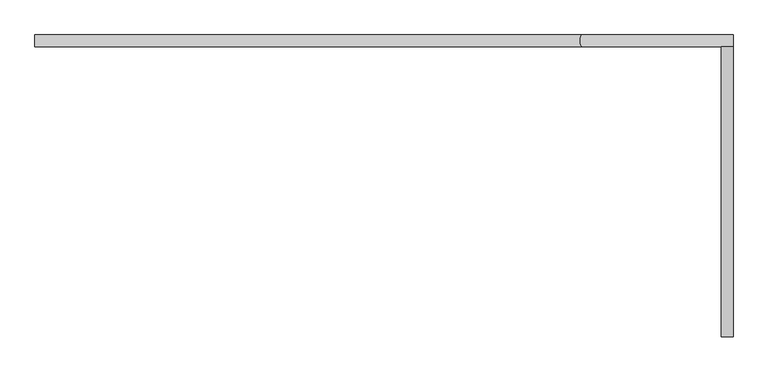
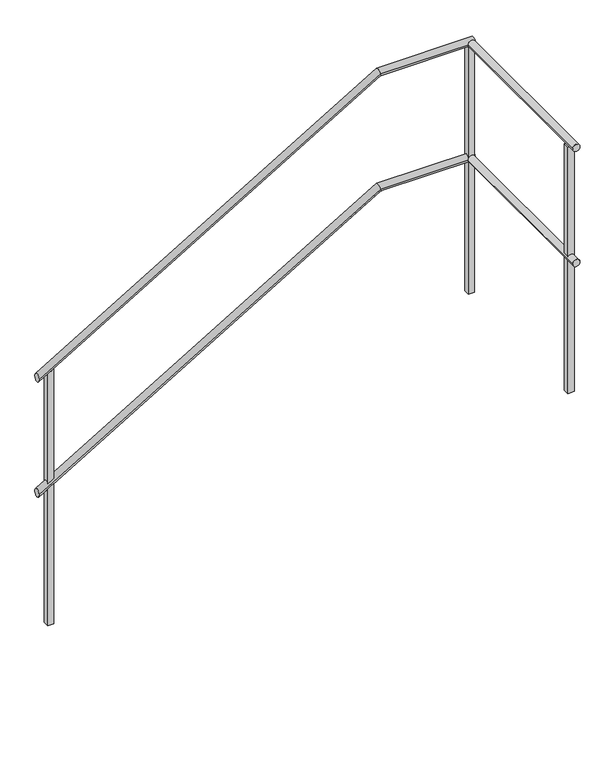
"""IFC4 building model written with IfcOpenShell, lengths in millimetres: railing geometry."""

from ifc_helpers import new_model, si_unit, frame, origin, place, context, project, spatial, polyline, circle_curve, ellipse_curve, outline, extrude, source, transform, mapped, element, save
from ifc_brep_helpers import plane_surface, cylinder_surface, advanced_brep


def railing_ac14cb65(model_context):
    return source(origin(), model_context, "Body", "SolidModel", [
        advanced_brep(
        [(43964.6, 23749.5208589, 1734.9618634), (43994.6, 23749.5208589, 1734.9618634), (43964.6, 24494.1208589, 1734.9618634), (43994.6, 24494.1208589, 1734.9618634)],
        [
            (0, 1, circle_curve(frame((43979.6, 23749.5208589, 1734.9618634), z_axis=(0.0, -1.0, 0.0), x_axis=(1.0, 0.0, 0.0)), 15.0)),
            (1, 0, circle_curve(frame((43979.6, 23749.5208589, 1734.9618634), z_axis=(0.0, -1.0, 0.0), x_axis=(1.0, 0.0, 0.0)), 15.0)),
            (2, 3, circle_curve(frame((43979.6, 24494.1208589, 1734.9618634), z_axis=(0.0, 1.0, 0.0), x_axis=(1.0, 0.0, 0.0)), 15.0)),
            (3, 2, circle_curve(frame((43979.6, 24494.1208589, 1734.9618634), z_axis=(0.0, 1.0, 0.0), x_axis=(1.0, 0.0, 0.0)), 15.0)),
            (0, 2),
            (3, 1),
        ],
        [
            plane_surface(frame((43979.6, 23749.5208589, 1749.9618634), z_axis=(0.0, -1.0, 0.0), x_axis=(0.0, 0.0, 1.0))),
            plane_surface(frame((43979.6, 24494.1208589, 1749.9618634), z_axis=(0.0, 1.0, 0.0), x_axis=(0.0, 0.0, 1.0))),
            cylinder_surface(frame((43979.6, 23749.5208589, 1734.9618634), z_axis=(0.0, -1.0, 0.0), x_axis=(1.0, 0.0, 0.0)), 15.0),
        ],
        [
            (0, [[1, 2]]),
            (1, [[3, 4]]),
            (2, [[-1, 5, -4, 6]]),
            (2, [[-2, -6, -3, -5]]),
        ],
    ),
        advanced_brep(
        [(43994.6, 24494.1208589, 1734.9618634), (43994.6, 24524.1208589, 1734.9618634), (43606.242552, 24494.1208589, 1734.9618634), (43606.242552, 24524.1208589, 1734.9618634), (42202.1161135, 24494.1208589, 899.1723166), (42202.1161135, 24524.1208589, 899.1723166)],
        [
            (0, 1, circle_curve(frame((43994.6, 24509.1208589, 1734.9618634), z_axis=(1.0, 0.0, 0.0), x_axis=(0.0, 1.0, 0.0)), 15.0)),
            (1, 0, circle_curve(frame((43994.6, 24509.1208589, 1734.9618634), z_axis=(1.0, 0.0, 0.0), x_axis=(0.0, 1.0, 0.0)), 15.0)),
            (0, 2),
            (2, 3, ellipse_curve(frame((43606.242552, 24509.1208589, 1734.9618634), z_axis=(0.9641817474962143, 0.0, 0.26524245096731114), x_axis=(0.265242450967311, 0.0, -0.9641817474962145)), 15.5572329, 15.0)),
            (3, 1),
            (3, 2, ellipse_curve(frame((43606.242552, 24509.1208589, 1734.9618634), z_axis=(0.9641817474962143, 0.0, 0.26524245096731114), x_axis=(0.265242450967311, 0.0, -0.9641817474962145)), 15.5572329, 15.0)),
            (4, 5, ellipse_curve(frame((42202.1161135, 24509.1208589, 899.1723166), z_axis=(-1.0, 0.0, 0.0), x_axis=(0.0, 0.0, 1.0)), 17.4562134, 15.0)),
            (5, 4, ellipse_curve(frame((42202.1161135, 24509.1208589, 899.1723166), z_axis=(-1.0, 0.0, 0.0), x_axis=(0.0, 0.0, 1.0)), 17.4562134, 15.0)),
            (2, 4),
            (5, 3),
        ],
        [
            plane_surface(frame((43994.6, 24509.1208589, 1749.9618634), z_axis=(1.0, 0.0, 0.0), x_axis=(0.0, -1.0, 0.0))),
            cylinder_surface(frame((43994.6, 24509.1208589, 1734.9618634), z_axis=(1.0, 0.0, 0.0), x_axis=(0.0, 1.0, 0.0)), 15.0),
            plane_surface(frame((42202.1161135, 24509.1208589, 916.62853), z_axis=(-1.0, 0.0, 0.0), x_axis=(0.0, -1.0, 0.0))),
            cylinder_surface(frame((43609.7883714, 24509.1208589, 1737.0724701), z_axis=(0.8592928844097072, 0.0, 0.511483859767682), x_axis=(0.0, 1.0, 0.0)), 15.0),
        ],
        [
            (0, [[1, 2]]),
            (1, [[-1, 3, 4, 5]]),
            (1, [[-2, -5, 6, -3]]),
            (2, [[7, 8]]),
            (3, [[-4, 9, -8, 10]]),
            (3, [[-6, -10, -7, -9]]),
        ],
    ),
        advanced_brep(
        [(43964.6, 23749.5208589, 2234.9618634), (43994.6, 23749.5208589, 2234.9618634), (43964.6, 24494.1208589, 2234.9618634), (43994.6, 24494.1208589, 2234.9618634)],
        [
            (0, 1, circle_curve(frame((43979.6, 23749.5208589, 2234.9618634), z_axis=(0.0, -1.0, 0.0), x_axis=(1.0, 0.0, 0.0)), 15.0)),
            (1, 0, circle_curve(frame((43979.6, 23749.5208589, 2234.9618634), z_axis=(0.0, -1.0, 0.0), x_axis=(1.0, 0.0, 0.0)), 15.0)),
            (2, 3, circle_curve(frame((43979.6, 24494.1208589, 2234.9618634), z_axis=(0.0, 1.0, 0.0), x_axis=(1.0, 0.0, 0.0)), 15.0)),
            (3, 2, circle_curve(frame((43979.6, 24494.1208589, 2234.9618634), z_axis=(0.0, 1.0, 0.0), x_axis=(1.0, 0.0, 0.0)), 15.0)),
            (0, 2),
            (3, 1),
        ],
        [
            plane_surface(frame((43979.6, 23749.5208589, 2249.9618634), z_axis=(0.0, -1.0, 0.0), x_axis=(0.0, 0.0, 1.0))),
            plane_surface(frame((43979.6, 24494.1208589, 2249.9618634), z_axis=(0.0, 1.0, 0.0), x_axis=(0.0, 0.0, 1.0))),
            cylinder_surface(frame((43979.6, 23749.5208589, 2234.9618634), z_axis=(0.0, -1.0, 0.0), x_axis=(1.0, 0.0, 0.0)), 15.0),
        ],
        [
            (0, [[1, 2]]),
            (1, [[3, 4]]),
            (2, [[-1, 5, -4, 6]]),
            (2, [[-2, -6, -3, -5]]),
        ],
    ),
        advanced_brep(
        [(43994.6, 24494.1208589, 2234.9618634), (43994.6, 24524.1208589, 2234.9618634), (43606.242552, 24494.1208589, 2234.9618634), (43606.242552, 24524.1208589, 2234.9618634), (42202.1161135, 24494.1208589, 1399.1723166), (42202.1161135, 24524.1208589, 1399.1723166)],
        [
            (0, 1, circle_curve(frame((43994.6, 24509.1208589, 2234.9618634), z_axis=(1.0, 0.0, 0.0), x_axis=(0.0, 1.0, 0.0)), 15.0)),
            (1, 0, circle_curve(frame((43994.6, 24509.1208589, 2234.9618634), z_axis=(1.0, 0.0, 0.0), x_axis=(0.0, 1.0, 0.0)), 15.0)),
            (0, 2),
            (2, 3, ellipse_curve(frame((43606.242552, 24509.1208589, 2234.9618634), z_axis=(0.9641817474962143, 0.0, 0.26524245096731114), x_axis=(0.265242450967311, 0.0, -0.9641817474962145)), 15.5572329, 15.0)),
            (3, 1),
            (3, 2, ellipse_curve(frame((43606.242552, 24509.1208589, 2234.9618634), z_axis=(0.9641817474962143, 0.0, 0.26524245096731114), x_axis=(0.265242450967311, 0.0, -0.9641817474962145)), 15.5572329, 15.0)),
            (4, 5, ellipse_curve(frame((42202.1161135, 24509.1208589, 1399.1723166), z_axis=(-1.0, 0.0, 0.0), x_axis=(0.0, 0.0, 1.0)), 17.4562134, 15.0)),
            (5, 4, ellipse_curve(frame((42202.1161135, 24509.1208589, 1399.1723166), z_axis=(-1.0, 0.0, 0.0), x_axis=(0.0, 0.0, 1.0)), 17.4562134, 15.0)),
            (2, 4),
            (5, 3),
        ],
        [
            plane_surface(frame((43994.6, 24509.1208589, 2249.9618634), z_axis=(1.0, 0.0, 0.0), x_axis=(0.0, -1.0, 0.0))),
            cylinder_surface(frame((43994.6, 24509.1208589, 2234.9618634), z_axis=(1.0, 0.0, 0.0), x_axis=(0.0, 1.0, 0.0)), 15.0),
            plane_surface(frame((42202.1161135, 24509.1208589, 1416.62853), z_axis=(-1.0, 0.0, 0.0), x_axis=(0.0, -1.0, 0.0))),
            cylinder_surface(frame((43609.7883714, 24509.1208589, 2237.0724701), z_axis=(0.8592928844097072, 0.0, 0.511483859767682), x_axis=(0.0, 1.0, 0.0)), 15.0),
        ],
        [
            (0, [[1, 2]]),
            (1, [[-1, 3, 4, 5]]),
            (1, [[-2, -5, 6, -3]]),
            (2, [[7, 8]]),
            (3, [[-4, 9, -8, 10]]),
            (3, [[-6, -10, -7, -9]]),
        ],
    ),
        extrude(outline(polyline([(43992.1, 24496.6208589), (43967.1, 24496.6208589), (43967.1, 24521.6208589), (43992.1, 24521.6208589), (43992.1, 24496.6208589)])), frame((0.0, 0.0, 1149.9618634), z_axis=(0.0, 0.0, 1.0), x_axis=(1.0, 0.0, 0.0)), (0.0, 0.0, 1.0), 1070.0),
        extrude(outline(polyline([(316.62853, 42264.6161135), (1423.830911, 42264.6161135), (1408.9499586, 42239.6161135), (316.62853, 42239.6161135), (316.62853, 42264.6161135)])), frame((0.0, 24496.6208589, 0.0), z_axis=(0.0, 1.0, 0.0), x_axis=(0.0, 0.0, 1.0)), (0.0, 0.0, 1.0), 25.0),
        extrude(outline(polyline([(43992.1, 23787.0208589), (43967.1, 23787.0208589), (43967.1, 23812.0208589), (43992.1, 23812.0208589), (43992.1, 23787.0208589)])), frame((0.0, 0.0, 1149.9618634), z_axis=(0.0, 0.0, 1.0), x_axis=(1.0, 0.0, 0.0)), (0.0, 0.0, 1.0), 1070.0),
    ])


if __name__ == "__main__":
    model = new_model("IFC4")
    model_context = context("Model", 3, world=origin())
    ifc_project = project(units=[si_unit("LENGTHUNIT", "METRE", prefix="MILLI")], contexts=[model_context])
    site = spatial("IfcSite", under=ifc_project)
    building = spatial("IfcBuilding", under=site)
    placement = place(None, origin())
    railing_shape = railing_ac14cb65(model_context)
    element("IfcRailing", 1, at=placement, inside=building, context=model_context, shape_type="MappedRepresentation", body=[
        mapped(railing_shape, transform((0.0, 0.0, 0.0), x_axis=(1.0, 0.0, 0.0), y_axis=(0.0, 1.0, 0.0), z_axis=(0.0, 0.0, 1.0))),
    ])
    save(model, "model.ifc")
